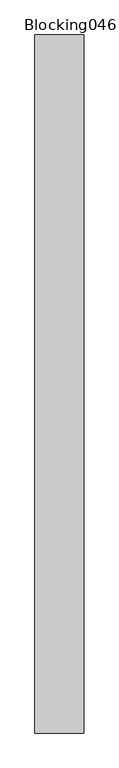
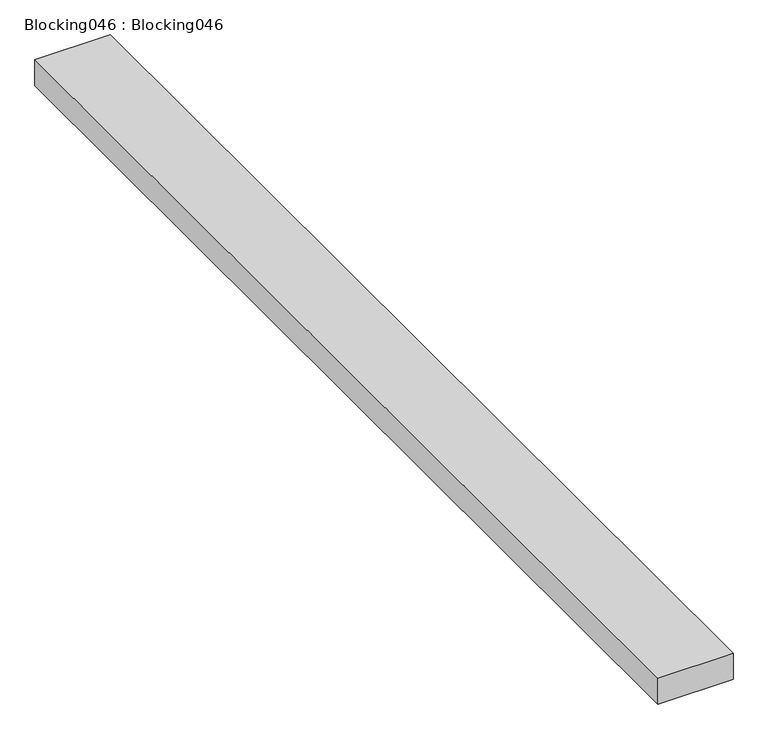
"""IFC4 building model written with IfcOpenShell, lengths in millimetres: proxy geometry, Blocking046 : Blocking046."""

from ifc_helpers import new_model, si_unit, frame, origin, place, context, project, spatial, polyline, outline, extrude, source, transform, mapped, element, save


def blocking046_blocking046_4b840a99(model_context):
    return source(origin(), model_context, "Body", "SweptSolid", [
        extrude(outline(polyline([(-950.3815411, -1052.8908936), (-1090.0815411, -1052.8908936), (-1090.0815411, 947.1091064), (-950.3815411, 947.1091064), (-950.3815411, -1052.8908936)])), frame((0.0, 0.0, 40163.496), z_axis=(0.0, 0.0, 1.0), x_axis=(1.0, 0.0, 0.0)), (0.0, 0.0, 1.0), 50.8),
    ])


if __name__ == "__main__":
    model = new_model("IFC4")
    model_context = context("Model", 3, world=origin())
    ifc_project = project(units=[si_unit("LENGTHUNIT", "METRE", prefix="MILLI")], contexts=[model_context])
    site = spatial("IfcSite", under=ifc_project)
    building = spatial("IfcBuilding", under=site)
    placement = place(None, origin())
    blocking046_blocking046_shape = blocking046_blocking046_4b840a99(model_context)
    element("IfcBuildingElementProxy", 1, Name="Blocking046 : Blocking046", ObjectType="Blocking046 : Blocking046", at=placement, inside=building, context=model_context, shape_type="MappedRepresentation", body=[
        mapped(blocking046_blocking046_shape, transform((0.0, 0.0, 0.0), x_axis=(1.0, 0.0, 0.0), y_axis=(0.0, 1.0, 0.0), z_axis=(0.0, 0.0, 1.0))),
    ])
    save(model, "model.ifc")

# Revit data of these elements
# Type "Blocking046 : Blocking046"
#   NameOverride = "Blocking046"
# Element 1 (IfcBuildingElementProxy, "Blocking046 : Blocking046")
#   Materials on its faces: "WOOD BLOCKING AS REQUIRED"
# Materials
#   "WOOD BLOCKING AS REQUIRED": class "Unassigned", colour RGB 166 124 85, transparency 0, Cost = 0
